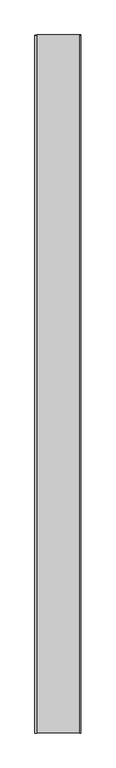
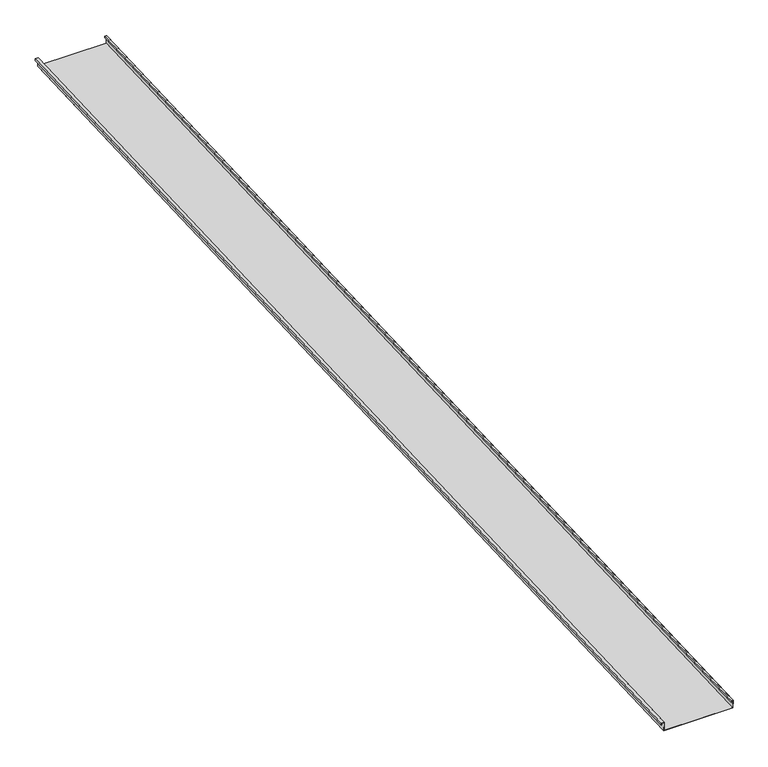
"""IFC4 building model written with IfcOpenShell, lengths in millimetres: proxy geometry, Generic Models 2:Generic Models 2:310765:Generic Models 2:310765 : Generic Models 2:Generic Models 2:310765:126 : Generic Models 2:Generic Models 2:310765:Generic Models 2:310765 : Generic Models 2:Generic Models 2:310765:300385."""

from ifc_helpers import new_model, si_unit, frame, origin, place, context, project, spatial, polyline, outline, extrude, source, transform, mapped, element, save


def generic_models_0f4a3aa8(model_context):
    return source(origin(), model_context, "Body", "SweptSolid", [
        extrude(outline(polyline([(1.5875, 0.0), (1.5875, 50.8), (407.9875, 50.8), (407.9875, 1.5875), (396.875, 1.5875), (396.875, 11.1125), (398.4625, 11.1125), (398.4625, 3.175), (406.4, 3.175), (406.4, 49.2125), (3.175, 49.2125), (3.175, -1.5874999), (-14.2875, -1.5874999), (-14.2875, 9.525), (-12.7, 9.525), (-12.7, 0.0), (1.5875, 0.0)])), frame((661349.9763072, -581354.4345603, 3902.6697972), z_axis=(0.0, 0.9991330730923568, 0.041630544712067834), x_axis=(1.0, 0.0, 0.0)), (0.0, 0.0, 1.0), 6400.8),
    ])


if __name__ == "__main__":
    model = new_model("IFC4")
    model_context = context("Model", 3, world=origin())
    ifc_project = project(units=[si_unit("LENGTHUNIT", "METRE", prefix="MILLI")], contexts=[model_context])
    site = spatial("IfcSite", under=ifc_project)
    building = spatial("IfcBuilding", under=site)
    placement = place(None, origin())
    generic_models_shape = generic_models_0f4a3aa8(model_context)
    element("IfcBuildingElementProxy", 1, Name="Generic Models 2:Generic Models 2:310765:Generic Models 2:310765 : Generic Models 2:Generic Models 2:310765:126 : Generic Models 2:Generic Models 2:310765:Generic Models 2:310765 : Generic Models 2:Generic Models 2:310765:300385", ObjectType="Generic Models 2:Generic Models 2:310765:Generic Models 2:310765 : Generic Models 2:Generic Models 2:310765:126 : Generic Models 2:Generic Models 2:310765:Generic Models 2:310765 : Generic Models 2:Generic Models 2:310765:300385", at=placement, inside=building, context=model_context, shape_type="MappedRepresentation", body=[
        mapped(generic_models_shape, transform((0.0, 0.0, 0.0), x_axis=(1.0, 0.0, 0.0), y_axis=(0.0, 1.0, 0.0), z_axis=(0.0, 0.0, 1.0))),
    ])
    save(model, "model.ifc")

# Revit data of these elements
# Type "Generic Models 2:Generic Models 2:310765:Generic Models 2:310765 : Generic Models 2:Generic Models 2:310765:126 : Generic Models 2:Generic Models 2:310765:Generic Models 2:310765 : Generic Models 2:Generic Models 2:310765:300385"
#   NameOverride = "Generic Models 2:Generic Models 2:310765:Generic Models 2:310765 : Generic Models 2:Generic Models 2:310765:300385"
#   ObjectTypeOverride = "Generic Models 2:310765 : Generic Models 2:Generic Models 2:310765"
#   Reference = "Generic Models 2"
#   Tag = "300385"
# Element 1 (IfcBuildingElementProxy, "Generic Models 2:Generic Models 2:310765:Generic Models 2:310765 : Generic Models 2:Generic Models 2:310765:126 : Generic Models 2:Generic Models 2:310765:Generic Models 2:310765 : Generic Models 2:Generic Models 2:310765:300385")
#   Materials on its faces: "THERMAL BROKEN ALUMINUM STOREFRONT FOR POLYCARBONATE"
# Materials
#   "THERMAL BROKEN ALUMINUM STOREFRONT FOR POLYCARBONATE": class "Unassigned", colour RGB 244 244 244, transparency 0, Keynote = "M07611300.01", Cost = 0
